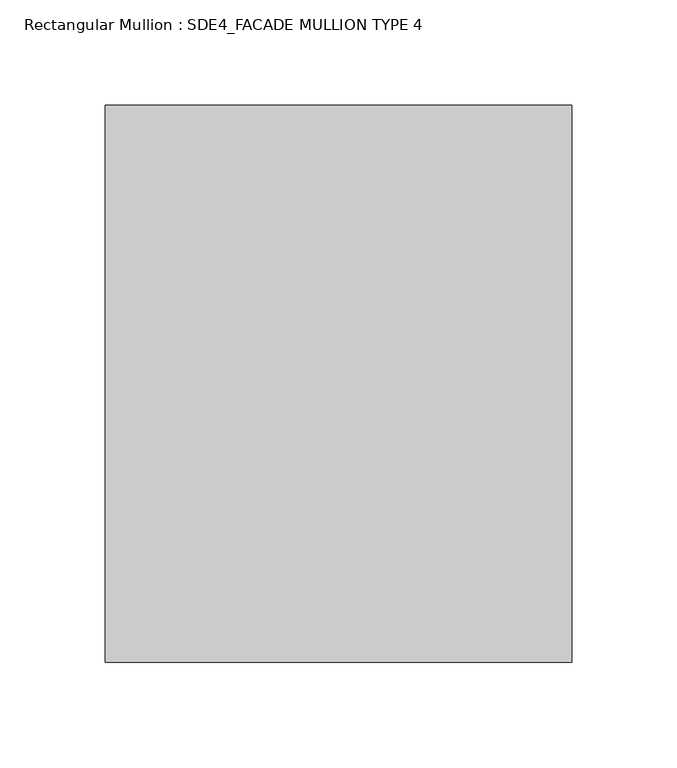
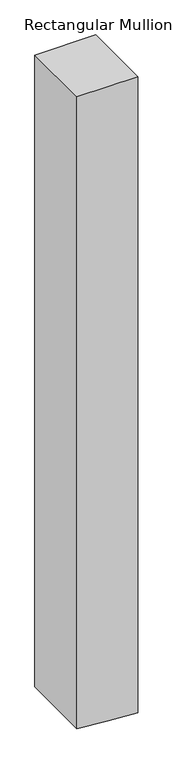
"""IFC4 building model written with IfcOpenShell, lengths in millimetres: member geometry, Rectangular Mullion : SDE4_FACADE MULLION TYPE 4."""

from ifc_helpers import new_model, si_unit, frame, origin, place, context, project, spatial, polyline, outline, extrude, source, transform, mapped, element, save


def rectangular_mullion_sde4_facade_mullion_type_4_ba65ab13(model_context):
    return source(origin(), model_context, "Body", "SweptSolid", [
        extrude(outline(polyline([(0.0, 111.0), (0.0, -111.0), (-2432.0142943, -111.0), (-2440.755216, 3.056508), (-2449.0276558, 111.0), (0.0, 111.0)])), frame((0.0, -132.5, 0.0), z_axis=(0.0, 1.0, 0.0), x_axis=(0.0, 0.0, 1.0)), (0.0, 0.0, 1.0), 265.0),
    ])


if __name__ == "__main__":
    model = new_model("IFC4")
    model_context = context("Model", 3, world=origin())
    ifc_project = project(units=[si_unit("LENGTHUNIT", "METRE", prefix="MILLI")], contexts=[model_context])
    site = spatial("IfcSite", under=ifc_project)
    building = spatial("IfcBuilding", under=site)
    placement = place(None, origin())
    rectangular_mullion_sde4_facade_mullion_type_4_shape = rectangular_mullion_sde4_facade_mullion_type_4_ba65ab13(model_context)
    element("IfcMember", 1, ObjectType="Rectangular Mullion : SDE4_FACADE MULLION TYPE 4", at=placement, inside=building, context=model_context, shape_type="MappedRepresentation", body=[
        mapped(rectangular_mullion_sde4_facade_mullion_type_4_shape, transform((0.0, 0.0, 0.0), x_axis=(1.0, 0.0, 0.0), y_axis=(0.0, 1.0, 0.0), z_axis=(0.0, 0.0, 1.0))),
    ])
    save(model, "model.ifc")

# Revit data of these elements
# Type "Rectangular Mullion : SDE4_FACADE MULLION TYPE 4"
#   built-in parameter 1007322 = 0.869423 (stored number, unit not read)
#   built-in parameter 1007321 = 0.364173 (stored number, unit not read)
#   built-in parameter 1007320 = 0.364173 (stored number, unit not read)
